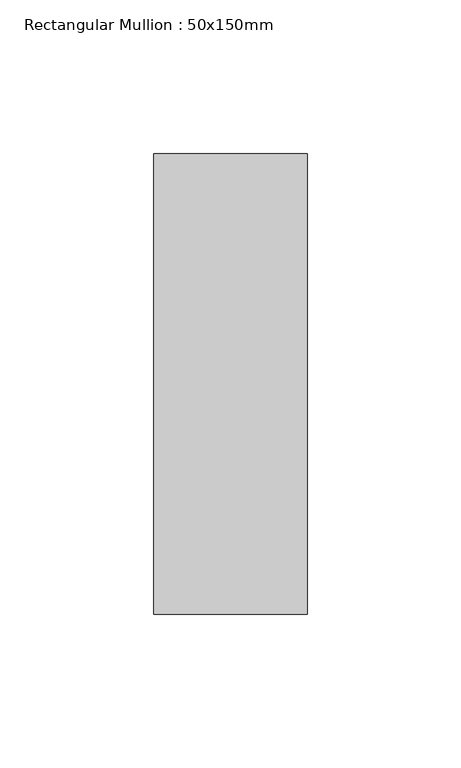
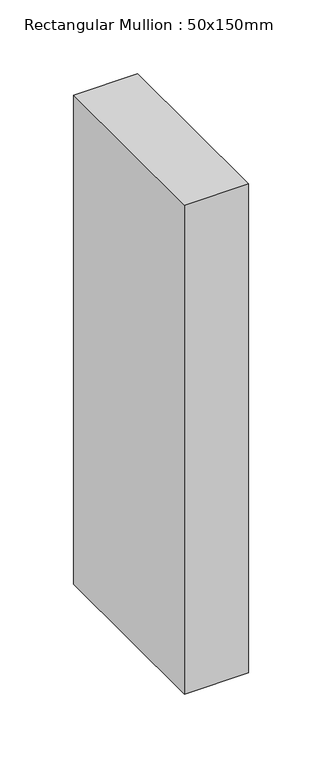
"""IFC4 building model written with IfcOpenShell, lengths in millimetres: member geometry, Rectangular Mullion : 50x150mm."""

from ifc_helpers import new_model, si_unit, frame, origin, place, context, project, spatial, polyline, outline, extrude, source, transform, mapped, element, save


def rectangular_mullion_50x150mm_e1d552ee(model_context):
    return source(origin(), model_context, "Body", "SweptSolid", [
        extrude(outline(polyline([(0.0, 75.0), (0.0, -75.0), (-50.0, -75.0), (-50.0, 75.0), (0.0, 75.0)])), frame((0.0, 0.0, -404.3238852), z_axis=(0.0, 0.0, 1.0), x_axis=(1.0, 0.0, 0.0)), (0.0, 0.0, 1.0), 404.3238852),
    ])


if __name__ == "__main__":
    model = new_model("IFC4")
    model_context = context("Model", 3, world=origin())
    ifc_project = project(units=[si_unit("LENGTHUNIT", "METRE", prefix="MILLI")], contexts=[model_context])
    site = spatial("IfcSite", under=ifc_project)
    building = spatial("IfcBuilding", under=site)
    placement = place(None, origin())
    rectangular_mullion_50x150mm_shape = rectangular_mullion_50x150mm_e1d552ee(model_context)
    element("IfcMember", 1, ObjectType="Rectangular Mullion : 50x150mm", at=placement, inside=building, context=model_context, shape_type="MappedRepresentation", body=[
        mapped(rectangular_mullion_50x150mm_shape, transform((0.0, 0.0, 0.0), x_axis=(1.0, 0.0, 0.0), y_axis=(0.0, 1.0, 0.0), z_axis=(0.0, 0.0, 1.0))),
    ])
    save(model, "model.ifc")

# Revit data of these elements
# Type "Rectangular Mullion : 50x150mm"
#   Keynote = "H11"
#   built-in parameter 1007304 = 0.492126 (stored number, unit not read)
#   built-in parameter 1007301 = 0.082021 (stored number, unit not read)
#   built-in parameter 1007300 = 0.082021 (stored number, unit not read)
# Element 1 (IfcMember, "Rectangular Mullion : 50x150mm")
#   Materials on its faces: "Aluminium"
# Materials
#   "Aluminium": class "Metal", colour RGB 247 247 247, transparency 0, Description = "Aluminium 6061", Cost = 0
